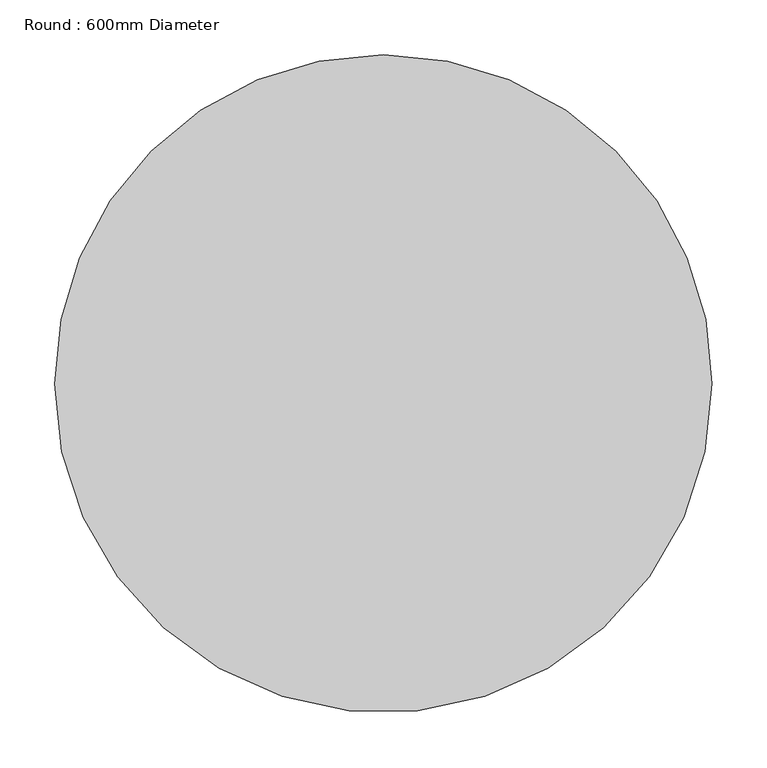
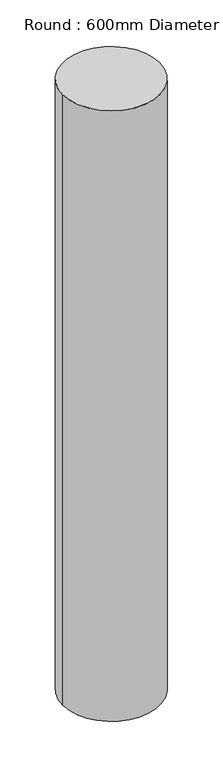
"""IFC4 building model written with IfcOpenShell, lengths in millimetres: column geometry, Round : 600mm Diameter."""

from ifc_helpers import new_model, si_unit, point, frame, origin, origin_2d, place, context, project, spatial, circle_curve, trimmed, segment, composite_curve, outline, extrude, source, transform, mapped, element, save


def round_600mm_diameter_3920c105(model_context):
    return source(origin(), model_context, "Body", "SweptSolid", [
        extrude(outline(composite_curve([segment(trimmed(circle_curve(origin_2d(), 300.0), [point((300.0, 0.0))], [point((-300.0, 0.0))], False, "CARTESIAN"), True, "CONTINUOUS"), segment(trimmed(circle_curve(origin_2d(), 300.0), [point((-300.0, 0.0))], [point((0.0, 300.0))], False, "CARTESIAN"), True, "CONTINUOUS"), segment(trimmed(circle_curve(origin_2d(), 300.0), [point((0.0, 300.0))], [point((300.0, 0.0))], False, "CARTESIAN"), True, "CONTINUOUS")], self_intersect=False)), frame((0.0, 0.0, 130470.0), z_axis=(0.0, 0.0, 1.0), x_axis=(1.0, 0.0, 0.0)), (0.0, 0.0, 1.0), 4000.0),
    ])


if __name__ == "__main__":
    model = new_model("IFC4")
    model_context = context("Model", 3, world=origin())
    ifc_project = project(units=[si_unit("LENGTHUNIT", "METRE", prefix="MILLI")], contexts=[model_context])
    site = spatial("IfcSite", under=ifc_project)
    building = spatial("IfcBuilding", under=site)
    placement = place(None, origin())
    round_600mm_diameter_shape = round_600mm_diameter_3920c105(model_context)
    element("IfcColumn", 1, ObjectType="Round : 600mm Diameter", at=placement, inside=building, context=model_context, shape_type="MappedRepresentation", body=[
        mapped(round_600mm_diameter_shape, transform((0.0, 0.0, 0.0), x_axis=(1.0, 0.0, 0.0), y_axis=(0.0, 1.0, 0.0), z_axis=(0.0, 0.0, 1.0))),
    ])
    save(model, "model.ifc")

# Revit data of these elements
# Type "Round : 600mm Diameter"
#   Keynote = "G"
#   Diameter = 600.00 mm
#   Offset Base = 0.00 mm
#   Offset Top = 0.00 mm
#   built-in parameter 1002110 = 8421504
#   built-in parameter 1002106 = element 3
#   Material = Concrete - Cast In Situ
# Element 1 (IfcColumn, "Round : 600mm Diameter")
#   Materials on its faces: "Concrete - Cast In Situ"
# Materials
#   "Concrete - Cast In Situ": class "Unassigned", colour RGB 255 255 255, transparency 0, Keynote = "E10/132", Cost = 0
